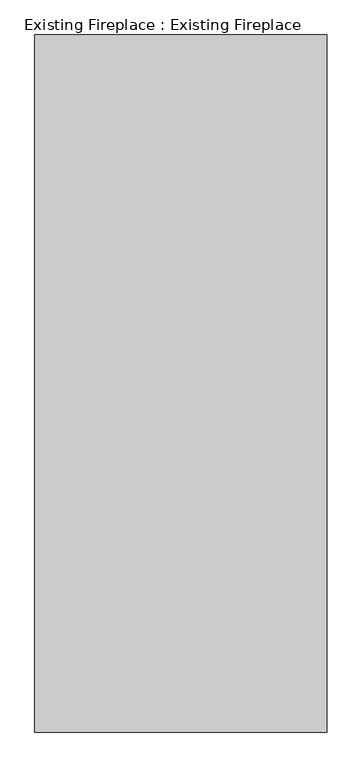
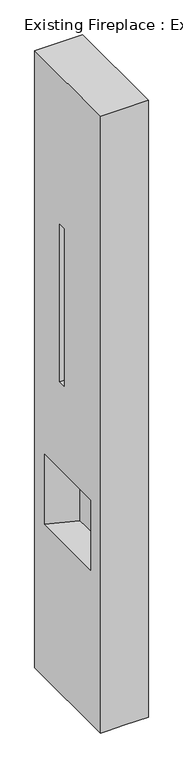
"""IFC4 building model written with IfcOpenShell, lengths in millimetres: proxy geometry, Existing Fireplace : Existing Fireplace."""

from ifc_helpers import new_model, si_unit, origin, place, context, project, spatial, faceted_brep, source, transform, mapped, element, save


def existing_fireplace_existing_fireplace_287aed51(model_context):
    return source(origin(), model_context, "Body", "Brep", [
        faceted_brep([(4450.2196932, 434.2888758, 8077.2), (3662.8196932, 434.2888758, 8077.2), (3662.8196932, -1445.3111242, 8077.2), (4450.2196932, -1445.3111242, 8077.2), (4450.2196932, 434.2888758, -2667.0), (4450.2196932, -1445.3111242, -2667.0), (4069.2196932, -1445.3111242, -2667.0), (3764.4196932, -1445.3111242, -2667.0), (3662.8196932, -1445.3111242, -2667.0), (3662.8196932, 434.2888758, -2667.0), (3764.4196932, 434.2888758, -2667.0), (4069.2196932, 434.2888758, -2667.0), (3662.8196932, 154.8888758, 0.0), (3662.8196932, 154.8888758, 1219.2), (3662.8196932, -1165.9111242, 1219.2), (3662.8196932, -1165.9111242, 0.0), (3662.8196932, -403.9111242, 5486.4), (3662.8196932, -403.9111242, 2743.2), (3662.8196932, -276.9111242, 2743.2), (3662.8196932, -276.9111242, 5486.4), (4145.4196932, -20.7631592, 1219.2), (4145.4196932, -990.2590891, 1219.2), (4145.4196932, -990.2590891, 0.0), (4145.4196932, -20.7631592, 0.0), (3767.2567114, -403.9111242, 5486.4), (3767.2567114, -403.9111242, 2743.2), (3767.2567114, -276.9111242, 2743.2), (3767.2567114, -276.9111242, 5486.4)], [[[0, 1, 2, 3]], [[4, 5, 6, 7, 8, 9, 10, 11]], [[1, 0, 4, 11, 10, 9]], [[2, 1, 9, 8], [12, 13, 14, 15], [16, 17, 18, 19]], [[3, 2, 8, 7, 6, 5]], [[0, 3, 5, 4]], [[14, 13, 20, 21]], [[15, 14, 21, 22]], [[21, 20, 23, 22]], [[13, 12, 23, 20]], [[12, 15, 22, 23]], [[24, 25, 17, 16]], [[26, 27, 19, 18]], [[25, 26, 18, 17]], [[25, 24, 27, 26]], [[27, 24, 16, 19]]]),
    ])


if __name__ == "__main__":
    model = new_model("IFC4")
    model_context = context("Model", 3, world=origin())
    ifc_project = project(units=[si_unit("LENGTHUNIT", "METRE", prefix="MILLI")], contexts=[model_context])
    site = spatial("IfcSite", under=ifc_project)
    building = spatial("IfcBuilding", under=site)
    placement = place(None, origin())
    existing_fireplace_existing_fireplace_shape = existing_fireplace_existing_fireplace_287aed51(model_context)
    element("IfcBuildingElementProxy", 1, Name="Existing Fireplace : Existing Fireplace", ObjectType="Existing Fireplace : Existing Fireplace", at=placement, inside=building, context=model_context, shape_type="MappedRepresentation", body=[
        mapped(existing_fireplace_existing_fireplace_shape, transform((0.0, 0.0, 0.0), x_axis=(1.0, 0.0, 0.0), y_axis=(0.0, 1.0, 0.0), z_axis=(0.0, 0.0, 1.0))),
    ])
    save(model, "model.ifc")

# Revit data of these elements
# Type "Existing Fireplace : Existing Fireplace"
#   Existing Brick = Brick, Existing
# Element 1 (IfcBuildingElementProxy, "Existing Fireplace : Existing Fireplace")
#   Materials on its faces: "Brick, Existing", "Concrete, Precast"
# Materials
#   "Brick, Existing": class "Masonry", colour RGB 137 111 95, transparency 0, Keynote = "04 21 00.A1", Description = "Common brick", Cost = 0
#   "Concrete, Precast": class "Concrete", colour RGB 198 187 187, transparency 0, Description = "Precast concrete", Cost = 0
